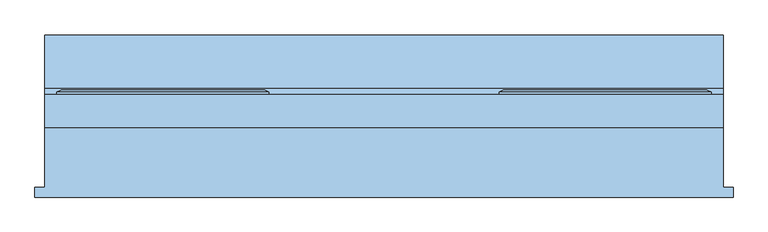
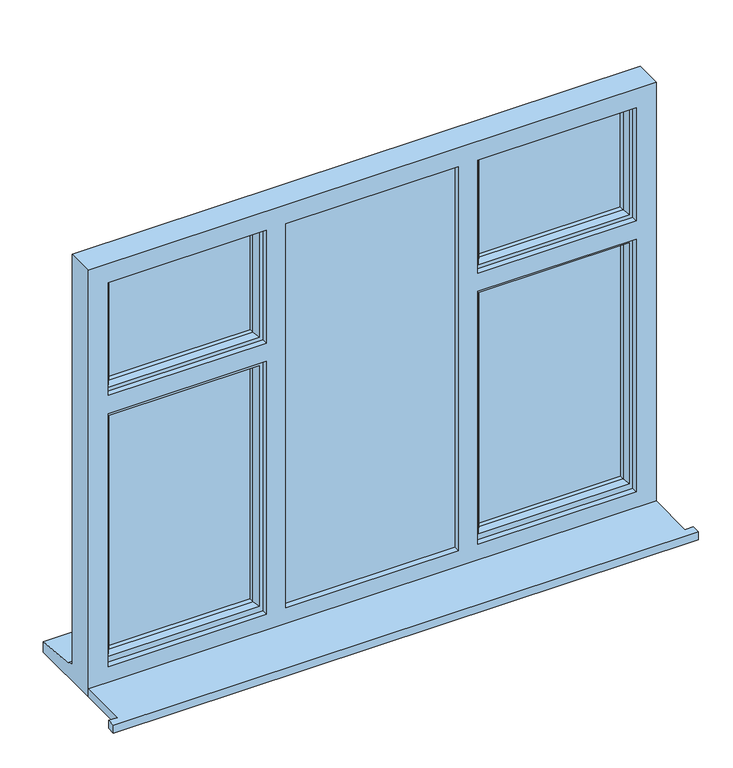
"""IFC4 building model written with IfcOpenShell, lengths in millimetres: window geometry, Window - Triple Casement with Top and Side Sashes : Window - Triple Casement with Top and Side Sashes 1700."""

from ifc_helpers import new_model, si_unit, frame, origin, place, context, project, spatial, polyline, outline, extrude, faceted_brep, source, transform, mapped, element, save


def window_acdad559(model_context):
    return source(origin(), model_context, "Body", "SolidModel", [
        extrude(outline(polyline([(-1433.3333333, -182.7934322), (-1433.3333333, -157.7934322), (-1408.3333333, -157.7934322), (-1408.3333333, -8.2934322), (291.6666667, -8.2934322), (291.6666667, -157.7934322), (316.6666667, -157.7934322), (316.6666667, -182.7934322), (-1433.3333333, -182.7934322)])), frame((0.0, 0.0, 760.0), z_axis=(0.0, 0.0, 1.0), x_axis=(1.0, 0.0, 0.0)), (0.0, 0.0, 1.0), 25.0),
        extrude(outline(polyline([(823.0, -826.6666667), (823.0, -290.0), (2070.0, -290.0), (2070.0, -826.6666667), (823.0, -826.6666667)]), holes=[polyline([(2060.0, -816.6666667), (2060.0, -300.0), (833.0, -300.0), (833.0, -816.6666667), (2060.0, -816.6666667)])]), frame((0.0, 33.7065678, 0.0), z_axis=(0.0, 1.0, 0.0), x_axis=(0.0, 0.0, 1.0)), (0.0, 0.0, 1.0), 41.0),
        faceted_brep([(-1378.3333333, 74.7065678, 2080.0), (-1378.3333333, 80.4800705, 2080.0), (-1378.3333333, 80.4800705, 1665.0), (-1378.3333333, 74.7065678, 1665.0), (-1368.3333333, 9.7065678, 2070.0), (-1368.3333333, 74.7065678, 2070.0), (-1368.3333333, 74.7065678, 1675.0), (-1368.3333333, 9.7065678, 1675.0), (-1328.3333333, 24.1994677, 2030.0), (-1338.4813711, 9.7065678, 2040.1480377), (-1338.4813711, 9.7065678, 1704.8519623), (-1328.3333333, 24.1994677, 1715.0), (-1328.3333333, 38.7065678, 2030.0), (-1328.3333333, 38.7065678, 1715.0), (-1338.3333333, 62.7065678, 2040.0), (-1338.3333333, 38.7065678, 2040.0), (-1338.3333333, 38.7065678, 1705.0), (-1338.3333333, 62.7065678, 1705.0), (-1328.3333333, 80.4800705, 2030.0), (-1328.3333333, 62.7065678, 2030.0), (-1328.3333333, 62.7065678, 1715.0), (-1328.3333333, 80.4800705, 1715.0), (-1345.7790881, 86.2535732, 2047.4457548), (-1345.7790881, 86.2535732, 1697.5542452), (-1367.5487236, 86.2535732, 2069.2153903), (-1367.5487236, 86.2535732, 1675.7846097), (-846.6666667, 80.4800705, 1665.0), (-846.6666667, 74.7065678, 1665.0), (-856.6666667, 74.7065678, 1675.0), (-856.6666667, 9.7065678, 1675.0), (-886.5186289, 9.7065678, 1704.8519623), (-896.6666667, 24.1994677, 1715.0), (-896.6666667, 38.7065678, 1715.0), (-886.6666667, 38.7065678, 1705.0), (-886.6666667, 62.7065678, 1705.0), (-896.6666667, 62.7065678, 1715.0), (-896.6666667, 80.4800705, 1715.0), (-879.2209119, 86.2535732, 1697.5542452), (-857.4512764, 86.2535732, 1675.7846097), (-846.6666667, 80.4800705, 2080.0), (-846.6666667, 74.7065678, 2080.0), (-856.6666667, 74.7065678, 2070.0), (-856.6666667, 9.7065678, 2070.0), (-886.5186289, 9.7065678, 2040.1480377), (-896.6666667, 24.1994677, 2030.0), (-896.6666667, 38.7065678, 2030.0), (-886.6666667, 38.7065678, 2040.0), (-886.6666667, 62.7065678, 2040.0), (-896.6666667, 62.7065678, 2030.0), (-896.6666667, 80.4800705, 2030.0), (-879.2209119, 86.2535732, 2047.4457548), (-857.4512764, 86.2535732, 2069.2153903)], [[[0, 1, 2, 3]], [[4, 5, 6, 7]], [[8, 9, 10, 11]], [[12, 8, 11, 13]], [[14, 15, 16, 17]], [[18, 19, 20, 21]], [[22, 18, 21, 23]], [[1, 24, 25, 2]], [[3, 2, 26, 27]], [[7, 6, 28, 29]], [[11, 10, 30, 31]], [[13, 11, 31, 32]], [[17, 16, 33, 34]], [[21, 20, 35, 36]], [[23, 21, 36, 37]], [[2, 25, 38, 26]], [[27, 26, 39, 40]], [[29, 28, 41, 42]], [[31, 30, 43, 44]], [[32, 31, 44, 45]], [[34, 33, 46, 47]], [[36, 35, 48, 49]], [[37, 36, 49, 50]], [[26, 38, 51, 39]], [[40, 39, 1, 0]], [[3, 27, 40, 0], [5, 41, 28, 6]], [[42, 41, 5, 4]], [[7, 29, 42, 4], [9, 43, 30, 10]], [[44, 43, 9, 8]], [[45, 44, 8, 12]], [[15, 46, 33, 16], [13, 32, 45, 12]], [[47, 46, 15, 14]], [[17, 34, 47, 14], [19, 48, 35, 20]], [[49, 48, 19, 18]], [[50, 49, 18, 22]], [[24, 51, 38, 25], [23, 37, 50, 22]], [[39, 51, 24, 1]]]),
        faceted_brep([(-1378.3333333, 74.7065678, 1655.0), (-1378.3333333, 80.4800705, 1655.0), (-1378.3333333, 80.4800705, 813.0), (-1378.3333333, 74.7065678, 813.0), (-1368.3333333, 9.7065678, 1645.0), (-1368.3333333, 74.7065678, 1645.0), (-1368.3333333, 74.7065678, 823.0), (-1368.3333333, 9.7065678, 823.0), (-1328.3333333, 24.1994677, 1605.0), (-1338.4813711, 9.7065678, 1615.1480377), (-1338.4813711, 9.7065678, 852.8519623), (-1328.3333333, 24.1994677, 863.0), (-1328.3333333, 38.7065678, 1605.0), (-1328.3333333, 38.7065678, 863.0), (-1338.3333333, 62.7065678, 1615.0), (-1338.3333333, 38.7065678, 1615.0), (-1338.3333333, 38.7065678, 853.0), (-1338.3333333, 62.7065678, 853.0), (-1328.3333333, 80.4800705, 1605.0), (-1328.3333333, 62.7065678, 1605.0), (-1328.3333333, 62.7065678, 863.0), (-1328.3333333, 80.4800705, 863.0), (-1345.7790881, 86.2535732, 1622.4457548), (-1345.7790881, 86.2535732, 845.5542452), (-1367.5487236, 86.2535732, 1644.2153903), (-1367.5487236, 86.2535732, 823.7846097), (-846.6666667, 80.4800705, 813.0), (-846.6666667, 74.7065678, 813.0), (-856.6666667, 74.7065678, 823.0), (-856.6666667, 9.7065678, 823.0), (-886.5186289, 9.7065678, 852.8519623), (-896.6666667, 24.1994677, 863.0), (-896.6666667, 38.7065678, 863.0), (-886.6666667, 38.7065678, 853.0), (-886.6666667, 62.7065678, 853.0), (-896.6666667, 62.7065678, 863.0), (-896.6666667, 80.4800705, 863.0), (-879.2209119, 86.2535732, 845.5542452), (-857.4512764, 86.2535732, 823.7846097), (-846.6666667, 80.4800705, 1655.0), (-846.6666667, 74.7065678, 1655.0), (-856.6666667, 74.7065678, 1645.0), (-856.6666667, 9.7065678, 1645.0), (-886.5186289, 9.7065678, 1615.1480377), (-896.6666667, 24.1994677, 1605.0), (-896.6666667, 38.7065678, 1605.0), (-886.6666667, 38.7065678, 1615.0), (-886.6666667, 62.7065678, 1615.0), (-896.6666667, 62.7065678, 1605.0), (-896.6666667, 80.4800705, 1605.0), (-879.2209119, 86.2535732, 1622.4457548), (-857.4512764, 86.2535732, 1644.2153903)], [[[0, 1, 2, 3]], [[4, 5, 6, 7]], [[8, 9, 10, 11]], [[12, 8, 11, 13]], [[14, 15, 16, 17]], [[18, 19, 20, 21]], [[22, 18, 21, 23]], [[1, 24, 25, 2]], [[3, 2, 26, 27]], [[7, 6, 28, 29]], [[11, 10, 30, 31]], [[13, 11, 31, 32]], [[17, 16, 33, 34]], [[21, 20, 35, 36]], [[23, 21, 36, 37]], [[2, 25, 38, 26]], [[27, 26, 39, 40]], [[29, 28, 41, 42]], [[31, 30, 43, 44]], [[32, 31, 44, 45]], [[34, 33, 46, 47]], [[36, 35, 48, 49]], [[37, 36, 49, 50]], [[26, 38, 51, 39]], [[40, 39, 1, 0]], [[3, 27, 40, 0], [5, 41, 28, 6]], [[42, 41, 5, 4]], [[7, 29, 42, 4], [9, 43, 30, 10]], [[44, 43, 9, 8]], [[45, 44, 8, 12]], [[15, 46, 33, 16], [13, 32, 45, 12]], [[47, 46, 15, 14]], [[17, 34, 47, 14], [19, 48, 35, 20]], [[49, 48, 19, 18]], [[50, 49, 18, 22]], [[24, 51, 38, 25], [23, 37, 50, 22]], [[39, 51, 24, 1]]]),
        faceted_brep([(-270.0, 74.7065678, 2080.0), (-270.0, 80.4800705, 2080.0), (-270.0, 80.4800705, 1665.0), (-270.0, 74.7065678, 1665.0), (-260.0, 9.7065678, 2070.0), (-260.0, 74.7065678, 2070.0), (-260.0, 74.7065678, 1675.0), (-260.0, 9.7065678, 1675.0), (-220.0, 24.1994677, 2030.0), (-230.1480377, 9.7065678, 2040.1480377), (-230.1480377, 9.7065678, 1704.8519623), (-220.0, 24.1994677, 1715.0), (-220.0, 38.7065678, 2030.0), (-220.0, 38.7065678, 1715.0), (-230.0, 62.7065678, 2040.0), (-230.0, 38.7065678, 2040.0), (-230.0, 38.7065678, 1705.0), (-230.0, 62.7065678, 1705.0), (-220.0, 80.4800705, 2030.0), (-220.0, 62.7065678, 2030.0), (-220.0, 62.7065678, 1715.0), (-220.0, 80.4800705, 1715.0), (-237.4457548, 86.2535732, 2047.4457548), (-237.4457548, 86.2535732, 1697.5542452), (-259.2153903, 86.2535732, 2069.2153903), (-259.2153903, 86.2535732, 1675.7846097), (261.6666667, 80.4800705, 1665.0), (261.6666667, 74.7065678, 1665.0), (251.6666667, 74.7065678, 1675.0), (251.6666667, 9.7065678, 1675.0), (221.8147044, 9.7065678, 1704.8519623), (211.6666667, 24.1994677, 1715.0), (211.6666667, 38.7065678, 1715.0), (221.6666667, 38.7065678, 1705.0), (221.6666667, 62.7065678, 1705.0), (211.6666667, 62.7065678, 1715.0), (211.6666667, 80.4800705, 1715.0), (229.1124215, 86.2535732, 1697.5542452), (250.882057, 86.2535732, 1675.7846097), (261.6666667, 80.4800705, 2080.0), (261.6666667, 74.7065678, 2080.0), (251.6666667, 74.7065678, 2070.0), (251.6666667, 9.7065678, 2070.0), (221.8147044, 9.7065678, 2040.1480377), (211.6666667, 24.1994677, 2030.0), (211.6666667, 38.7065678, 2030.0), (221.6666667, 38.7065678, 2040.0), (221.6666667, 62.7065678, 2040.0), (211.6666667, 62.7065678, 2030.0), (211.6666667, 80.4800705, 2030.0), (229.1124215, 86.2535732, 2047.4457548), (250.882057, 86.2535732, 2069.2153903)], [[[0, 1, 2, 3]], [[4, 5, 6, 7]], [[8, 9, 10, 11]], [[12, 8, 11, 13]], [[14, 15, 16, 17]], [[18, 19, 20, 21]], [[22, 18, 21, 23]], [[1, 24, 25, 2]], [[3, 2, 26, 27]], [[7, 6, 28, 29]], [[11, 10, 30, 31]], [[13, 11, 31, 32]], [[17, 16, 33, 34]], [[21, 20, 35, 36]], [[23, 21, 36, 37]], [[2, 25, 38, 26]], [[27, 26, 39, 40]], [[29, 28, 41, 42]], [[31, 30, 43, 44]], [[32, 31, 44, 45]], [[34, 33, 46, 47]], [[36, 35, 48, 49]], [[37, 36, 49, 50]], [[26, 38, 51, 39]], [[40, 39, 1, 0]], [[3, 27, 40, 0], [5, 41, 28, 6]], [[42, 41, 5, 4]], [[7, 29, 42, 4], [9, 43, 30, 10]], [[44, 43, 9, 8]], [[45, 44, 8, 12]], [[15, 46, 33, 16], [13, 32, 45, 12]], [[47, 46, 15, 14]], [[17, 34, 47, 14], [19, 48, 35, 20]], [[49, 48, 19, 18]], [[50, 49, 18, 22]], [[24, 51, 38, 25], [23, 37, 50, 22]], [[39, 51, 24, 1]]]),
        extrude(outline(polyline([(221.6666667, 38.7065678), (-230.1480377, 38.7065678), (-230.1480377, 62.7065678), (221.6666667, 62.7065678), (221.6666667, 38.7065678)])), frame((0.0, 0.0, 852.8519623), z_axis=(0.0, 0.0, 1.0), x_axis=(1.0, 0.0, 0.0)), (0.0, 0.0, 1.0), 762.1480377),
        extrude(outline(polyline([(221.6666667, 38.7065678), (-230.0, 38.7065678), (-230.0, 62.7065678), (221.6666667, 62.7065678), (221.6666667, 38.7065678)])), frame((0.0, 0.0, 1705.0), z_axis=(0.0, 0.0, 1.0), x_axis=(1.0, 0.0, 0.0)), (0.0, 0.0, 1.0), 335.0),
        extrude(outline(polyline([(-886.6666667, 38.7065678), (-1338.3333333, 38.7065678), (-1338.3333333, 62.7065678), (-886.6666667, 62.7065678), (-886.6666667, 38.7065678)])), frame((0.0, 0.0, 1705.0), z_axis=(0.0, 0.0, 1.0), x_axis=(1.0, 0.0, 0.0)), (0.0, 0.0, 1.0), 335.0),
        extrude(outline(polyline([(-886.6666667, 38.7065678), (-1338.3333333, 38.7065678), (-1338.3333333, 62.7065678), (-886.6666667, 62.7065678), (-886.6666667, 38.7065678)])), frame((0.0, 0.0, 853.0), z_axis=(0.0, 0.0, 1.0), x_axis=(1.0, 0.0, 0.0)), (0.0, 0.0, 1.0), 762.0),
        faceted_brep([(-270.0, 74.7065678, 1655.0), (-270.0, 80.4800705, 1655.0), (-270.0, 80.4800705, 813.0), (-270.0, 74.7065678, 813.0), (-260.0, 9.7065678, 1645.0), (-260.0, 74.7065678, 1645.0), (-260.0, 74.7065678, 823.0), (-260.0, 9.7065678, 823.0), (-220.0, 24.1994677, 1605.0), (-230.1480377, 9.7065678, 1615.1480377), (-230.1480377, 9.7065678, 852.8519623), (-220.0, 24.1994677, 863.0), (-220.0, 38.7065678, 1605.0), (-220.0, 38.7065678, 863.0), (-230.0, 62.7065678, 1615.0), (-230.0, 38.7065678, 1615.0), (-230.0, 38.7065678, 853.0), (-230.0, 62.7065678, 853.0), (-220.0, 80.4800705, 1605.0), (-220.0, 62.7065678, 1605.0), (-220.0, 62.7065678, 863.0), (-220.0, 80.4800705, 863.0), (-237.4457548, 86.2535732, 1622.4457548), (-237.4457548, 86.2535732, 845.5542452), (-259.2153903, 86.2535732, 1644.2153903), (-259.2153903, 86.2535732, 823.7846097), (261.6666667, 80.4800705, 813.0), (261.6666667, 74.7065678, 813.0), (251.6666667, 74.7065678, 823.0), (251.6666667, 9.7065678, 823.0), (221.8147044, 9.7065678, 852.8519623), (211.6666667, 24.1994677, 863.0), (211.6666667, 38.7065678, 863.0), (221.6666667, 38.7065678, 853.0), (221.6666667, 62.7065678, 853.0), (211.6666667, 62.7065678, 863.0), (211.6666667, 80.4800705, 863.0), (229.1124215, 86.2535732, 845.5542452), (250.882057, 86.2535732, 823.7846097), (261.6666667, 80.4800705, 1655.0), (261.6666667, 74.7065678, 1655.0), (251.6666667, 74.7065678, 1645.0), (251.6666667, 9.7065678, 1645.0), (221.8147044, 9.7065678, 1615.1480377), (211.6666667, 24.1994677, 1605.0), (211.6666667, 38.7065678, 1605.0), (221.6666667, 38.7065678, 1615.0), (221.6666667, 62.7065678, 1615.0), (211.6666667, 62.7065678, 1605.0), (211.6666667, 80.4800705, 1605.0), (229.1124215, 86.2535732, 1622.4457548), (250.882057, 86.2535732, 1644.2153903)], [[[0, 1, 2, 3]], [[4, 5, 6, 7]], [[8, 9, 10, 11]], [[12, 8, 11, 13]], [[14, 15, 16, 17]], [[18, 19, 20, 21]], [[22, 18, 21, 23]], [[1, 24, 25, 2]], [[3, 2, 26, 27]], [[7, 6, 28, 29]], [[11, 10, 30, 31]], [[13, 11, 31, 32]], [[17, 16, 33, 34]], [[21, 20, 35, 36]], [[23, 21, 36, 37]], [[2, 25, 38, 26]], [[27, 26, 39, 40]], [[29, 28, 41, 42]], [[31, 30, 43, 44]], [[32, 31, 44, 45]], [[34, 33, 46, 47]], [[36, 35, 48, 49]], [[37, 36, 49, 50]], [[26, 38, 51, 39]], [[40, 39, 1, 0]], [[3, 27, 40, 0], [5, 41, 28, 6]], [[42, 41, 5, 4]], [[7, 29, 42, 4], [9, 43, 30, 10]], [[44, 43, 9, 8]], [[45, 44, 8, 12]], [[15, 46, 33, 16], [13, 32, 45, 12]], [[47, 46, 15, 14]], [[17, 34, 47, 14], [19, 48, 35, 20]], [[49, 48, 19, 18]], [[50, 49, 18, 22]], [[24, 51, 38, 25], [23, 37, 50, 22]], [[39, 51, 24, 1]]]),
        faceted_brep([(291.6666667, -8.2934322, 2110.0), (-1408.3333333, -8.2934322, 2110.0), (-1408.3333333, -8.2934322, 760.0), (291.6666667, -8.2934322, 760.0), (231.6666667, -8.2934322, 835.0), (-242.0, -8.2934322, 835.0), (-242.0, -8.2934322, 1635.0), (231.6666667, -8.2934322, 1635.0), (-816.6666667, -8.2934322, 2050.0), (-300.0, -8.2934322, 2050.0), (-300.0, -8.2934322, 835.0), (-816.6666667, -8.2934322, 835.0), (-242.0, -8.2934322, 2050.0), (231.6666667, -8.2934322, 2050.0), (231.6666667, -8.2934322, 1693.0), (-242.0, -8.2934322, 1693.0), (-1348.3333333, -8.2934322, 835.0), (-1348.3333333, -8.2934322, 1635.0), (-874.6666667, -8.2934322, 1635.0), (-874.6666667, -8.2934322, 835.0), (-1348.3333333, -8.2934322, 2050.0), (-874.6666667, -8.2934322, 2050.0), (-874.6666667, -8.2934322, 1693.0), (-1348.3333333, -8.2934322, 1693.0), (-1408.3333333, 74.7065678, 2110.0), (-1408.3333333, 74.7065678, 811.0), (-1408.3333333, 89.7065678, 809.68767), (-1408.3333333, 89.7065678, 804.7449676), (-1408.3333333, 224.7065678, 793.8088847), (-1408.3333333, 224.7065678, 760.0), (291.6666667, 74.7065678, 2110.0), (291.6666667, 74.7065678, 811.0), (-260.0, 74.7065678, 823.0), (251.6666667, 74.7065678, 823.0), (251.6666667, 74.7065678, 1645.0), (-260.0, 74.7065678, 1645.0), (251.6666667, 74.7065678, 2070.0), (-260.0, 74.7065678, 2070.0), (-260.0, 74.7065678, 1675.0), (251.6666667, 74.7065678, 1675.0), (-856.6666667, 74.7065678, 823.0), (-856.6666667, 74.7065678, 1645.0), (-1368.3333333, 74.7065678, 1645.0), (-1368.3333333, 74.7065678, 823.0), (-856.6666667, 74.7065678, 2070.0), (-1368.3333333, 74.7065678, 2070.0), (-1368.3333333, 74.7065678, 1675.0), (-856.6666667, 74.7065678, 1675.0), (-816.6666667, 74.7065678, 2070.0), (-816.6666667, 74.7065678, 823.0), (-300.0, 74.7065678, 823.0), (-300.0, 74.7065678, 2070.0), (-1368.3333333, 9.7065678, 2070.0), (-1368.3333333, 9.7065678, 1675.0), (-1368.3333333, 9.7065678, 1645.0), (-1368.3333333, 9.7065678, 823.0), (-856.6666667, 9.7065678, 2070.0), (-856.6666667, 9.7065678, 1675.0), (-874.6666667, 9.7065678, 2050.0), (-1348.3333333, 9.7065678, 2050.0), (-1348.3333333, 9.7065678, 1693.0), (-874.6666667, 9.7065678, 1693.0), (-260.0, 9.7065678, 2070.0), (251.6666667, 9.7065678, 2070.0), (251.6666667, 9.7065678, 1675.0), (-260.0, 9.7065678, 1675.0), (231.6666667, 9.7065678, 2050.0), (-242.0, 9.7065678, 2050.0), (-242.0, 9.7065678, 1693.0), (231.6666667, 9.7065678, 1693.0), (-826.6666667, 9.7065678, 2070.0), (-290.0, 9.7065678, 2070.0), (-290.0, 9.7065678, 823.0), (-826.6666667, 9.7065678, 823.0), (-300.0, 9.7065678, 2050.0), (-816.6666667, 9.7065678, 2050.0), (-816.6666667, 9.7065678, 835.0), (-300.0, 9.7065678, 835.0), (-856.6666667, 9.7065678, 823.0), (-856.6666667, 9.7065678, 1645.0), (-1348.3333333, 9.7065678, 835.0), (-874.6666667, 9.7065678, 835.0), (-874.6666667, 9.7065678, 1635.0), (-1348.3333333, 9.7065678, 1635.0), (251.6666667, 9.7065678, 823.0), (-260.0, 9.7065678, 823.0), (-260.0, 9.7065678, 1645.0), (251.6666667, 9.7065678, 1645.0), (-242.0, 9.7065678, 835.0), (231.6666667, 9.7065678, 835.0), (231.6666667, 9.7065678, 1635.0), (-242.0, 9.7065678, 1635.0), (-816.6666667, 33.7065678, 2070.0), (-300.0, 33.7065678, 2070.0), (-290.0, 33.7065678, 2070.0), (-826.6666667, 33.7065678, 2070.0), (291.6666667, 224.7065678, 760.0), (291.6666667, 224.7065678, 793.8088847), (291.6666667, 89.7065678, 804.7449676), (291.6666667, 89.7065678, 809.68767), (-816.6666667, 33.7065678, 823.0), (-826.6666667, 33.7065678, 823.0), (-290.0, 33.7065678, 823.0), (-300.0, 33.7065678, 823.0)], [[[0, 1, 2, 3], [4, 5, 6, 7], [8, 9, 10, 11], [12, 13, 14, 15], [16, 17, 18, 19], [20, 21, 22, 23]], [[1, 24, 25, 26, 27, 28, 29, 2]], [[24, 30, 31, 25], [32, 33, 34, 35], [36, 37, 38, 39], [40, 41, 42, 43], [44, 45, 46, 47], [48, 49, 50, 51]], [[45, 52, 53, 46]], [[54, 55, 43, 42]], [[52, 56, 57, 53], [58, 59, 60, 61]], [[62, 63, 64, 65], [66, 67, 68, 69]], [[70, 71, 72, 73], [74, 75, 76, 77]], [[78, 55, 54, 79], [80, 81, 82, 83]], [[84, 85, 86, 87], [88, 89, 90, 91]], [[59, 20, 23, 60]], [[16, 80, 83, 17]], [[1, 0, 30, 24]], [[52, 45, 44, 56]], [[36, 63, 62, 37]], [[92, 48, 51, 93, 94, 71, 70, 95]], [[20, 59, 58, 21]], [[66, 13, 12, 67]], [[8, 75, 74, 9]], [[30, 0, 3, 96, 97, 98, 99, 31]], [[63, 36, 39, 64]], [[33, 84, 87, 34]], [[13, 66, 69, 14]], [[89, 4, 7, 90]], [[75, 8, 11, 76]], [[21, 58, 61, 22]], [[81, 19, 18, 82]], [[57, 56, 44, 47]], [[40, 78, 79, 41]], [[49, 48, 92, 100]], [[100, 92, 95, 101]], [[101, 95, 70, 73]], [[94, 102, 72, 71]], [[102, 94, 93, 103]], [[103, 93, 51, 50]], [[37, 62, 65, 38]], [[85, 32, 35, 86]], [[67, 12, 15, 68]], [[5, 88, 91, 6]], [[9, 74, 77, 10]], [[96, 3, 2, 29]], [[97, 96, 29, 28]], [[98, 97, 28, 27]], [[99, 98, 27, 26]], [[31, 99, 26, 25]], [[33, 32, 85, 84]], [[40, 43, 55, 78]], [[50, 49, 100, 101, 73, 72, 102, 103]], [[5, 4, 89, 88]], [[77, 76, 11, 10]], [[81, 80, 16, 19]], [[35, 34, 87, 86]], [[39, 38, 65, 64]], [[15, 14, 69, 68]], [[7, 6, 91, 90]], [[47, 46, 53, 57]], [[42, 41, 79, 54]], [[83, 82, 18, 17]], [[61, 60, 23, 22]]]),
        extrude(outline(polyline([(-826.6666667, 33.7065678), (-290.0, 33.7065678), (-290.0, 9.7065678), (-826.6666667, 9.7065678), (-826.6666667, 33.7065678)])), frame((0.0, 0.0, 823.0), z_axis=(0.0, 0.0, 1.0), x_axis=(1.0, 0.0, 0.0)), (0.0, 0.0, 1.0), 1247.0),
    ])


if __name__ == "__main__":
    model = new_model("IFC4")
    model_context = context("Model", 3, world=origin())
    ifc_project = project(units=[si_unit("LENGTHUNIT", "METRE", prefix="MILLI")], contexts=[model_context])
    site = spatial("IfcSite", under=ifc_project)
    building = spatial("IfcBuilding", under=site)
    placement = place(None, origin())
    window_shape = window_acdad559(model_context)
    element("IfcWindow", 1, ObjectType="Window - Triple Casement with Top and Side Sashes : Window - Triple Casement with Top and Side Sashes 1700", at=placement, inside=building, context=model_context, shape_type="MappedRepresentation", body=[
        mapped(window_shape, transform((0.0, 0.0, 0.0), x_axis=(1.0, 0.0, 0.0), y_axis=(0.0, 1.0, 0.0), z_axis=(0.0, 0.0, 1.0))),
    ])
    save(model, "model.ifc")

# Revit data of these elements
# Type "Window - Triple Casement with Top and Side Sashes : Window - Triple Casement with Top and Side Sashes 1700"
#   Description = "Triple Casement Window with Opening Sash Vents"
#   Type Mark = "60"
#   Operation = "Userdefined"
#   Manufacturer = "Revit"
#   Keynote = "L10"
#   Wrap Layers (Ext) from Ext = 100 mm
#   Wrap Layers (Int) from Ext = 177.5 mm
#   Window Board Projection = 25 mm
#   Window Board Extension = 25 mm
#   Visual Light Transmittance = 0.9
#   Vent Height = 450 mm
#   Solar Heat Gain Coefficient = 0.78
#   Rough Width = 1700 mm
#   Rough Height = 1350 mm
#   Height = 1350 mm
#   Width = 1700 mm
#   Heat Transfer Coefficient (U) = 3.6886 W/(m²·K)
#   Glazing Thickness = 24 mm
#   FrameOffset - External = 100 mm
#   Frame Depth = 65 mm
#   Default Head Height = 2110 mm
#   Cill Depth = 150 mm
#   Cavity Closer Width = 50 mm
#   Cavity Closer Offset from Ext = 102.5 mm
#   Cavity Closer Depth = 85 mm
#   Vis - Cavity Closers = yes
#   Material Trim = Window Frame
#   Material Glass = Glass
#   Material Frame = Window Frame
#   Construction Type Id = ""
#   Wall Closure = (empty or 0)
#   Analytic Construction = (empty or 0)
# Element 1 (IfcWindow, "Window - Triple Casement with Top and Side Sashes : Window - Triple Casement with Top and Side Sashes 1700")
#   Materials on its faces: "Window Frame", "Glass"
# Materials
#   "Window Frame": class "Miscellaneous", colour RGB 249 249 249, transparency 0, Keynote = "L10"
#   "Glass": class "Glass", colour RGB 0 128 192, transparency 0.9, Description = "Soda Lime Glass", Cost = 0
